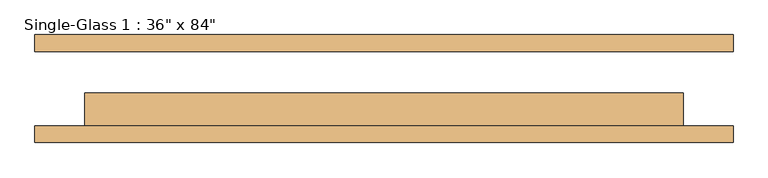
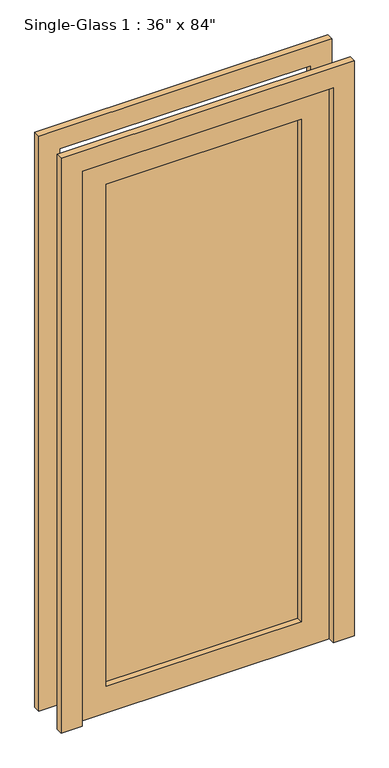
"""IFC4 building model written with IfcOpenShell, lengths in millimetres: door geometry."""

from ifc_helpers import new_model, si_unit, frame, origin, place, context, project, spatial, polyline, outline, extrude, source, transform, mapped, element, save


def door_d71a8095(model_context):
    return source(origin(), model_context, "Body", "SweptSolid", [
        extrude(outline(polyline([(2133.6, 457.2), (0.0, 457.2), (0.0, 533.4), (2209.8, 533.4), (2209.8, -533.4), (0.0, -533.4), (0.0, -457.2), (2133.6, -457.2), (2133.6, 457.2)])), frame((0.0, 57.15, 0.0), z_axis=(0.0, 1.0, 0.0), x_axis=(0.0, 0.0, 1.0)), (0.0, 0.0, 1.0), 25.4),
        extrude(outline(polyline([(2133.6, 457.2), (0.0, 457.2), (0.0, 533.4), (2209.8, 533.4), (2209.8, -533.4), (0.0, -533.4), (0.0, -457.2), (2133.6, -457.2), (2133.6, 457.2)])), frame((0.0, -82.55, 0.0), z_axis=(0.0, 1.0, 0.0), x_axis=(0.0, 0.0, 1.0)), (0.0, 0.0, 1.0), 25.4),
        extrude(outline(polyline([(355.6, -28.575), (355.6, -34.925), (-355.6, -34.925), (-355.6, -28.575), (355.6, -28.575)])), frame((0.0, 0.0, 101.6), z_axis=(0.0, 0.0, 1.0), x_axis=(1.0, 0.0, 0.0)), (0.0, 0.0, 1.0), 1930.4),
        extrude(outline(polyline([(2133.6, 457.2), (2133.6, -457.2), (0.0, -457.2), (0.0, 457.2), (2133.6, 457.2)]), holes=[polyline([(2032.0, -355.6), (2032.0, 355.6), (101.6, 355.6), (101.6, -355.6), (2032.0, -355.6)])]), frame((0.0, -57.15, 0.0), z_axis=(0.0, 1.0, 0.0), x_axis=(0.0, 0.0, 1.0)), (0.0, 0.0, 1.0), 50.8),
    ])


if __name__ == "__main__":
    model = new_model("IFC4")
    model_context = context("Model", 3, world=origin())
    ifc_project = project(units=[si_unit("LENGTHUNIT", "METRE", prefix="MILLI")], contexts=[model_context])
    site = spatial("IfcSite", under=ifc_project)
    building = spatial("IfcBuilding", under=site)
    placement = place(None, origin())
    door_shape = door_d71a8095(model_context)
    element("IfcDoor", 1, ObjectType="Single-Glass 1 : 36\" x 84\"", at=placement, inside=building, context=model_context, shape_type="MappedRepresentation", body=[
        mapped(door_shape, transform((0.0, 0.0, 0.0), x_axis=(1.0, 0.0, 0.0), y_axis=(0.0, 1.0, 0.0), z_axis=(0.0, 0.0, 1.0))),
    ])
    save(model, "model.ifc")

# Revit data of these elements
# Type "Single-Glass 1 : 36\" x 84\""
#   Type Mark = "27"
#   Assembly Code = "C1020"
#   Thickness = 0' - 2"
#   Height = 7' - 0"
#   Rail Width - Base = 0' - 4"
#   Rail Width - Top = 0' - 4"
#   Stile Width - Hinge = 0' - 4"
#   Stile Width - Latch = 0' - 4"
#   Trim Projection Ext = 0' - 1"
#   Trim Projection Int = 0' - 1"
#   Trim Width = 0' - 3"
#   Width = 3' - 0"
#   Function = 0
#   Door Material = Door - Panel
#   Frame Material = Door - Frame
#   Wall Closure = (empty or 0)
# Element 1 (IfcDoor, "Single-Glass 1 : 36\" x 84\"")
#   Materials on its faces: "Door - Frame", "Door - Panel", "Glass"
# Materials
#   "Door - Panel": class "Wood", colour RGB 230 193 158, transparency 0, Cost = 0
#   "Door - Frame": class "Paint", colour RGB 113 0 0, transparency 0, Cost = 0
#   "Glass": class "Glass", colour RGB 0 128 192, transparency 0.75, Cost = 0
